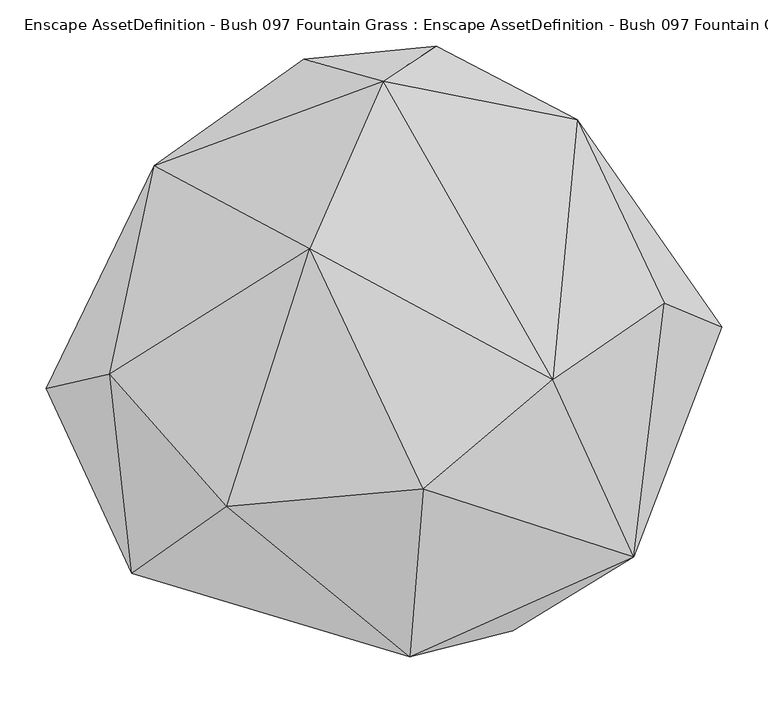
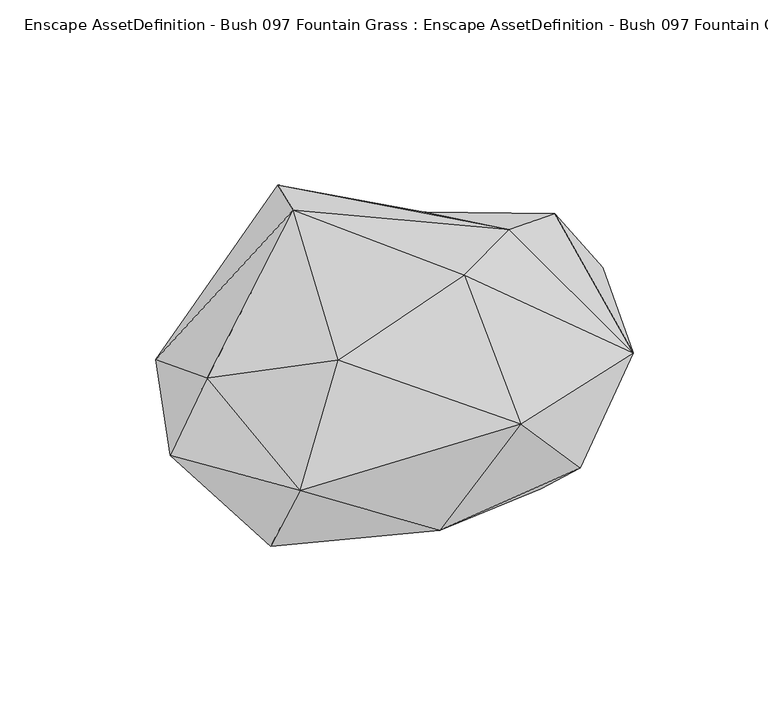
"""IFC4 building model written with IfcOpenShell, lengths in millimetres: geographic element geometry, Enscape AssetDefinition - Bush 097 Fountain Grass : Enscape AssetDefinition - Bush 097 Fountain Grass."""

from ifc_helpers import new_model, si_unit, origin, place, context, project, spatial, faceted_brep, source, transform, mapped, element, save


def enscape_assetdefinition_bush_097_fountain_grass_enscape_1502b8b9(model_context):
    return source(origin(), model_context, "Body", "Brep", [
        faceted_brep([(-261.6530061, 207.9070061, 157.3020071), (-100.1069993, 322.8589892, 164.4250005), (-160.1630002, 64.6440014, 0.0), (57.847999, 185.4089946, 0.0), (43.1380011, 337.033987, 178.332001), (-14.246, 299.3960083, 309.4969988), (209.4389945, 80.7560012, 0.0), (195.0130016, 257.8909993, 216.5929973), (168.9170003, -23.0960008, 365.8989966), (-93.6670005, 118.6890006, 405.0750136), (288.9080048, 59.6019998, 301.214993), (351.1109948, 33.7780006, 204.0619999), (155.7759941, -133.0550015, 0.0), (256.1340034, -214.3449932, 243.2319969), (28.7970006, -141.3120031, 410.5660021), (-182.9980016, -160.2070034, 352.1730006), (-309.6390069, -17.1000008, 279.8430026), (14.1399996, -322.2959936, 273.6000121), (125.6390065, -294.6949899, 143.8259929), (-285.7509851, -232.5409949, 212.1620029), (-87.7140015, -274.7980058, 100.8519977), (-378.0399859, -32.7499993, 182.0120066), (-236.6909981, -66.9969991, 0.0)], [[[0, 1, 2]], [[1, 3, 2]], [[1, 4, 3]], [[5, 4, 1]], [[1, 0, 5]], [[3, 6, 2]], [[3, 7, 6]], [[3, 4, 7]], [[7, 4, 5]], [[7, 5, 8]], [[5, 0, 9]], [[8, 5, 9]], [[10, 7, 8]], [[10, 11, 7]], [[11, 6, 7]], [[6, 12, 2]], [[6, 11, 12]], [[10, 13, 11]], [[11, 13, 12]], [[13, 10, 8]], [[14, 13, 8]], [[14, 8, 9]], [[14, 9, 15]], [[9, 16, 15]], [[0, 16, 9]], [[14, 15, 17]], [[17, 13, 14]], [[13, 18, 12]], [[17, 18, 13]], [[15, 19, 17]], [[19, 20, 17]], [[17, 20, 18]], [[15, 16, 19]], [[21, 16, 0]], [[21, 19, 16]], [[22, 0, 2]], [[21, 0, 22]], [[21, 22, 19]], [[19, 22, 20]], [[20, 22, 12]], [[20, 12, 18]], [[12, 22, 2]]]),
    ])


if __name__ == "__main__":
    model = new_model("IFC4")
    model_context = context("Model", 3, world=origin())
    ifc_project = project(units=[si_unit("LENGTHUNIT", "METRE", prefix="MILLI")], contexts=[model_context])
    site = spatial("IfcSite", under=ifc_project)
    building = spatial("IfcBuilding", under=site)
    placement = place(None, origin())
    enscape_assetdefinition_bush_097_fountain_grass_enscape_shape = enscape_assetdefinition_bush_097_fountain_grass_enscape_1502b8b9(model_context)
    element("IfcGeographicElement", 1, ObjectType="Enscape AssetDefinition - Bush 097 Fountain Grass : Enscape AssetDefinition - Bush 097 Fountain Grass", at=placement, inside=building, context=model_context, shape_type="MappedRepresentation", body=[
        mapped(enscape_assetdefinition_bush_097_fountain_grass_enscape_shape, transform((0.0, 0.0, 0.0), x_axis=(1.0, 0.0, 0.0), y_axis=(0.0, 1.0, 0.0), z_axis=(0.0, 0.0, 1.0))),
    ])
    save(model, "model.ifc")

# Revit data of these elements
# Type "Enscape AssetDefinition - Bush 097 Fountain Grass : Enscape AssetDefinition - Bush 097 Fountain Grass"
#   EnscapeAssetSource = "REMOTE"
#   EnscapeAssetId = "598bd5e1-d5d2-440b-8bd4-0d63a2768afb"
#   Height = 0.410566 m
#   EnscapeNativeAssetHeight = 0.410566 m
#   Default Elevation = 0
